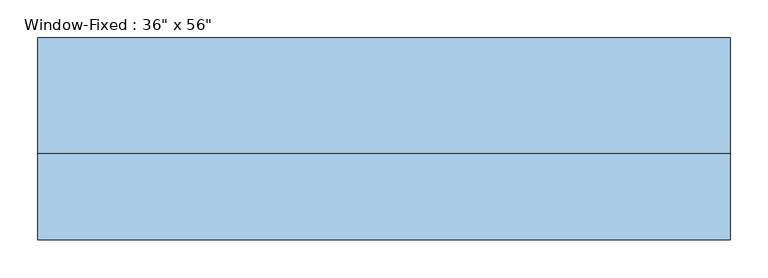
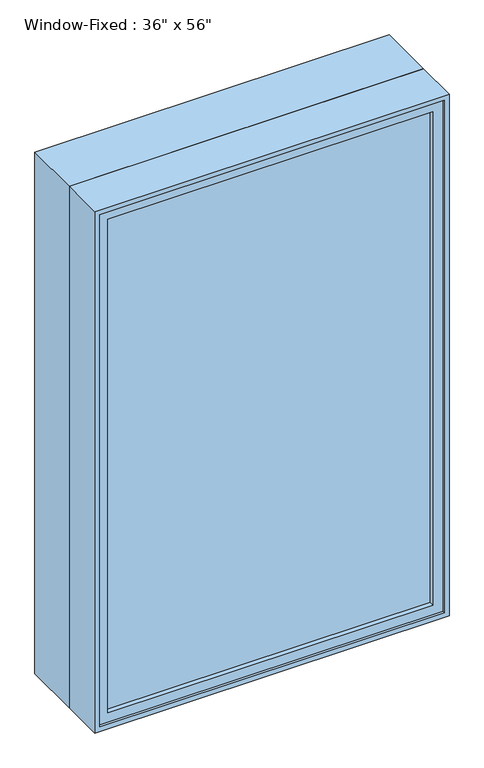
"""IFC4 building model written with IfcOpenShell, lengths in millimetres: window geometry."""

from ifc_helpers import new_model, si_unit, frame, origin, place, context, project, spatial, polyline, outline, extrude, faceted_brep, source, transform, mapped, element, save


def window_66a382c3(model_context):
    return source(origin(), model_context, "Body", "SolidModel", [
        extrude(outline(polyline([(419.1, -79.375), (-419.1, -79.375), (-419.1, -73.025), (419.1, -73.025), (419.1, -79.375)])), frame((0.0, 0.0, 952.5), z_axis=(0.0, 0.0, 1.0), x_axis=(1.0, 0.0, 0.0)), (0.0, 0.0, 1.0), 1346.2),
        extrude(outline(polyline([(-419.1, -60.325), (419.1, -60.325), (419.1, -66.675), (-419.1, -66.675), (-419.1, -60.325)])), frame((0.0, 0.0, 952.5), z_axis=(0.0, 0.0, 1.0), x_axis=(1.0, 0.0, 0.0)), (0.0, 0.0, 1.0), 1346.2),
        extrude(outline(polyline([(927.1, -444.5), (927.1, 444.5), (2324.1, 444.5), (2324.1, -444.5), (927.1, -444.5)]), holes=[polyline([(952.5, 419.1), (952.5, -419.1), (2298.7, -419.1), (2298.7, 419.1), (952.5, 419.1)])]), frame((0.0, -92.075, 0.0), z_axis=(0.0, 1.0, 0.0), x_axis=(0.0, 0.0, 1.0)), (0.0, 0.0, 1.0), 44.45),
        extrude(outline(polyline([(2336.8, -457.2), (914.4, -457.2), (914.4, 457.2), (2336.8, 457.2), (2336.8, -457.2)]), holes=[polyline([(2324.1, 444.5), (927.1, 444.5), (927.1, -444.5), (2324.1, -444.5), (2324.1, 444.5)])]), frame((0.0, 15.875, 0.0), z_axis=(0.0, 1.0, 0.0), x_axis=(0.0, 0.0, 1.0)), (0.0, 0.0, 1.0), 152.4),
        faceted_brep([(457.2, 15.875, 2336.8), (-457.2, 15.875, 2336.8), (-457.2, -98.425, 2336.8), (457.2, -98.425, 2336.8), (-457.2, 15.875, 914.4), (-457.2, -98.425, 914.4), (457.2, 15.875, 914.4), (457.2, -98.425, 914.4), (425.45, 15.875, 2305.05), (-425.45, 15.875, 2305.05), (-425.45, 15.875, 946.15), (425.45, 15.875, 946.15), (-444.5, -98.425, 2324.1), (444.5, -98.425, 2324.1), (444.5, -98.425, 927.1), (-444.5, -98.425, 927.1), (425.45, -47.625, 2305.05), (-425.45, -47.625, 2305.05), (-444.5, -47.625, 2324.1), (444.5, -47.625, 2324.1), (-425.45, -47.625, 946.15), (-444.5, -47.625, 927.1), (425.45, -47.625, 946.15), (444.5, -47.625, 927.1)], [[[0, 1, 2, 3]], [[1, 4, 5, 2]], [[4, 6, 7, 5]], [[1, 0, 6, 4], [8, 9, 10, 11]], [[6, 0, 3, 7]], [[3, 2, 5, 7], [12, 13, 14, 15]], [[16, 17, 9, 8]], [[13, 12, 18, 19]], [[17, 20, 10, 9]], [[12, 15, 21, 18]], [[20, 22, 11, 10]], [[15, 14, 23, 21]], [[22, 16, 8, 11]], [[19, 18, 21, 23], [17, 16, 22, 20]], [[14, 13, 19, 23]]]),
    ])


if __name__ == "__main__":
    model = new_model("IFC4")
    model_context = context("Model", 3, world=origin())
    ifc_project = project(units=[si_unit("LENGTHUNIT", "METRE", prefix="MILLI")], contexts=[model_context])
    site = spatial("IfcSite", under=ifc_project)
    building = spatial("IfcBuilding", under=site)
    placement = place(None, origin())
    window_shape = window_66a382c3(model_context)
    element("IfcWindow", 1, ObjectType="Window-Fixed : 36\" x 56\"", at=placement, inside=building, context=model_context, shape_type="MappedRepresentation", body=[
        mapped(window_shape, transform((0.0, 0.0, 0.0), x_axis=(1.0, 0.0, 0.0), y_axis=(0.0, 1.0, 0.0), z_axis=(0.0, 0.0, 1.0))),
    ])
    save(model, "model.ifc")

# Revit data of these elements
# Type "Window-Fixed : 36\" x 56\""
#   Type Mark = "22"
#   Fire Rating = "0.5h"
#   Assembly Code = "B2020100"
#   Analytic Construction = "Double glazing - domestic"
#   Window Inset [instance default] = 0' - 0"
#   Wall Thickness [instance default] = 0' - 6"
#   Visual Light Transmittance = 0.81
#   Thermal Resistance (R) = 1.8146 (h·ft²·°F)/BTU
#   Solar Heat Gain Coefficient = 0.76
#   Rough Width = 3' - 0 1/2"
#   Rough Height = 4' - 8 1/2"
#   Interior Wall Closure [instance default] = 0' - 2 1/4"
#   Height = 4' - 8"
#   Heat Transfer Coefficient (U) = 0.5511 BTU/(h·ft²·°F)
#   Frame Extension [instance default] = 0' - 0 1/4"
#   Exterior Wall Closure [instance default] = 0' - 1 1/4"
#   Extension Jamb [instance default] = 0' - 2 1/4"
#   Default Sill Height = 3' - 0"
#   Width = 3' - 0"
#   Muntin Visibility = yes
#   Interior Trim Visibility [instance default] = yes
#   Exterior Trim Visibility [instance default] = yes
#   Extension Jamb Visibility [instance default] = yes
#   Muntin Pattern = Muntin Pattern_2x2 : Muntin Pattern_2x2
#   Interior Trim Material = Wood - Stained
#   Interior Trim = Trim-Window-Interior-Flat : Picture Frame
#   Interior Frame Material = Wood - Stained
#   Glass Panel Material = Glass
#   Exterior Trim Material = Clad - White
#   Exterior Trim = Trim-Window-Exterior-Flat : with Sill
#   Exterior Frame Material = Clad - White
#   Wall Closure = (empty or 0)
# Element 1 (IfcWindow, "Window-Fixed : 36\" x 56\"")
#   Window Inset = 0' - 3 1/2"
#   Wall Thickness = 1' - 1 1/4"
#   Exterior Wall Closure = 0' - 5 1/2"
#   Extension Jamb = 0' - 6"
#   Exterior Trim Visibility = no
#   Materials on its faces: "Wood - Stained", "Glass", "Clad - White"
# Materials
#   "Wood - Stained": class "Wood", colour RGB 224 178 126, transparency 0, Cost = 0
#   "Glass": class "Glass", colour RGB 0 128 192, transparency 0.75, Description = "Soda Lime Glass", Cost = 0
#   "Clad - White": class "Wood", colour RGB 242 242 238, transparency 0, Cost = 0
